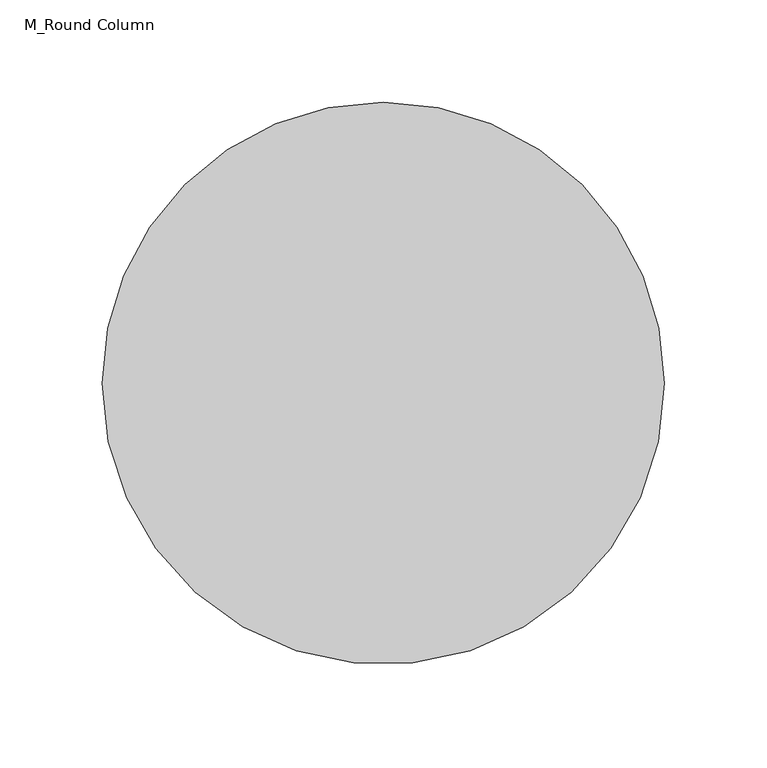
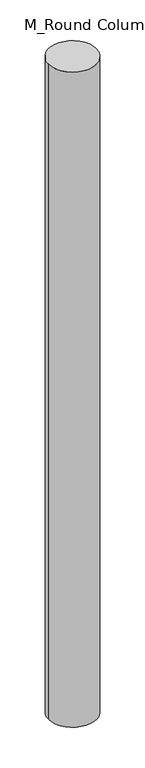
"""IFC4 building model written with IfcOpenShell, lengths in millimetres: column geometry, M_Round Column : 275mm DiameteR."""

from ifc_helpers import new_model, si_unit, point, origin, origin_with_axes, origin_2d, place, context, project, spatial, circle_curve, trimmed, segment, composite_curve, outline, extrude, source, transform, mapped, element, save


def m_round_column_1d8452c1(model_context):
    return source(origin(), model_context, "Body", "SweptSolid", [
        extrude(outline(composite_curve([segment(trimmed(circle_curve(origin_2d(), 137.5), [point((137.5, 0.0))], [point((-137.5, 0.0))], False, "CARTESIAN"), True, "CONTINUOUS"), segment(trimmed(circle_curve(origin_2d(), 137.5), [point((-137.5, 0.0))], [point((0.0, 137.5))], False, "CARTESIAN"), True, "CONTINUOUS"), segment(trimmed(circle_curve(origin_2d(), 137.5), [point((0.0, 137.5))], [point((137.5, 0.0))], False, "CARTESIAN"), True, "CONTINUOUS")], self_intersect=False)), origin_with_axes(), (0.0, 0.0, 1.0), 4000.0),
    ])


if __name__ == "__main__":
    model = new_model("IFC4")
    model_context = context("Model", 3, world=origin())
    ifc_project = project(units=[si_unit("LENGTHUNIT", "METRE", prefix="MILLI")], contexts=[model_context])
    site = spatial("IfcSite", under=ifc_project)
    building = spatial("IfcBuilding", under=site)
    placement = place(None, origin())
    m_round_column_shape = m_round_column_1d8452c1(model_context)
    element("IfcColumn", 1, ObjectType="M_Round Column : 275mm DiameteR", at=placement, inside=building, context=model_context, shape_type="MappedRepresentation", body=[
        mapped(m_round_column_shape, transform((0.0, 0.0, 0.0), x_axis=(1.0, 0.0, 0.0), y_axis=(0.0, 1.0, 0.0), z_axis=(0.0, 0.0, 1.0))),
    ])
    save(model, "model.ifc")

# Revit data of these elements
# Type "M_Round Column : 275mm DiameteR"
#   Diameter = 275 mm
#   Offset Base = 0 mm
#   Offset Top = 0 mm
#   COBie.Type = no
#   Material = none
